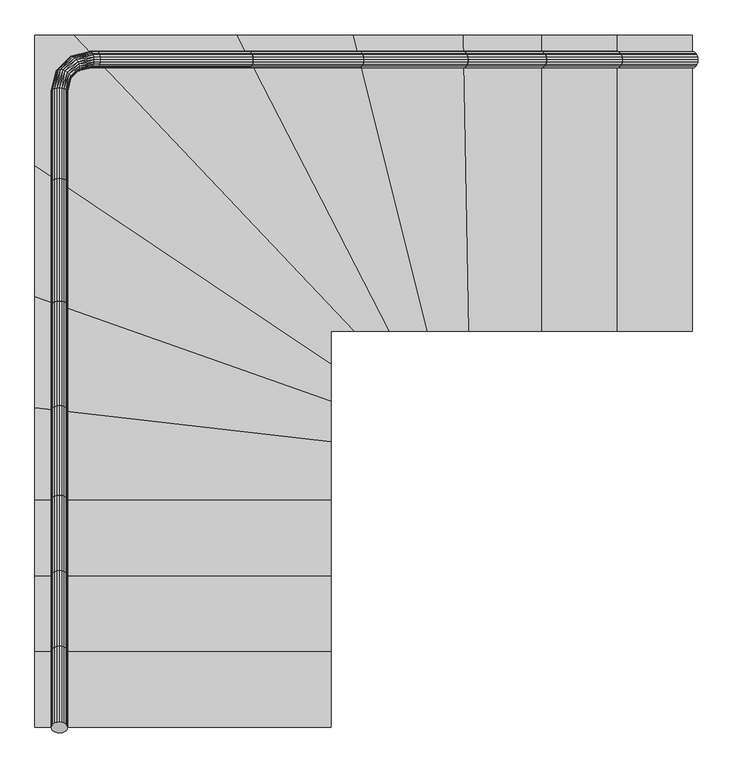
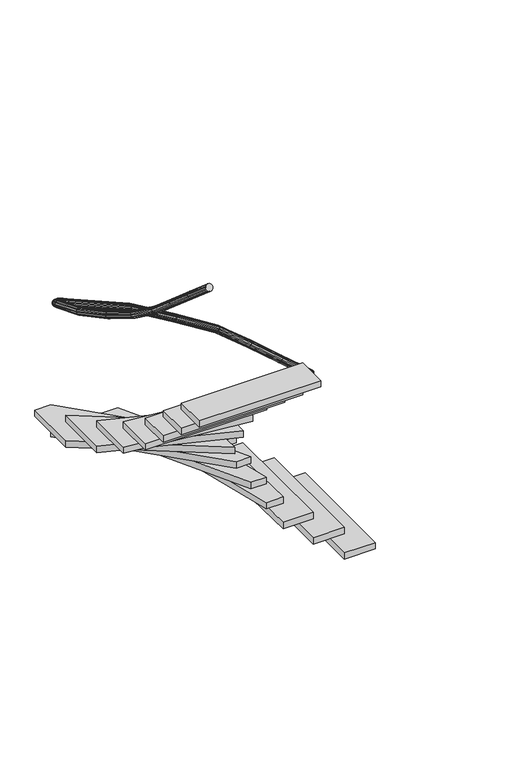
"""IFC4 building model written with IfcOpenShell, lengths in millimetres: stair geometry, 0_3d_modell."""

from ifc_helpers import new_model, si_unit, frame, origin, origin_with_axes, place, context, project, spatial, polyline, outline, extrude, faceted_brep, source, transform, mapped, element, save


def stair_5a7e43e8(model_context):
    return source(origin(), model_context, "Body", "SolidModel", [
        extrude(outline(polyline([(0.0, 988.8933271), (900.0, 884.9103911), (900.0, 706.9018591), (0.0, 706.9018591), (0.0, 988.8933271)])), frame((0.0, 0.0, 1787.1428571), z_axis=(0.0, 0.0, 1.0), x_axis=(1.0, 0.0, 0.0)), (0.0, 0.0, 1.0), 50.0),
        extrude(outline(polyline([(1.2235871, -7.9923214), (0.0, 0.0), (1.2235871, 7.9923214), (4.7745751, 15.2022986), (10.3053687, 20.924169), (17.2745751, 24.597836), (25.0, 25.8636953), (32.7254249, 24.597836), (39.6946313, 20.924169), (45.2254249, 15.2022986), (48.7764129, 7.9923214), (50.0, 0.0), (48.7764129, -7.9923214), (45.2254249, -15.2022986), (39.6946313, -20.924169), (32.7254249, -24.5978359), (25.0, -25.8636953), (17.2745751, -24.5978359), (10.3053687, -20.924169), (4.7745751, -15.2022986), (1.2235871, -7.9923214)])), frame((100.0, 246.9018591, 3252.4163795), z_axis=(0.0, -0.7569287102856999, 0.653497457948558), x_axis=(-1.0, 0.0, 0.0)), (0.0, 0.0, 1.0), 303.8595272),
        faceted_brep([(1775.2229617, 2022.7272828, 1074.1802827), (1770.0, 2021.5036957, 1068.1306652), (1764.7770383, 2022.7272828, 1062.0810477), (1760.0653365, 2026.2782709, 1056.6236089), (1756.3261087, 2031.8090644, 1052.2925609), (1753.9253768, 2038.7782709, 1049.511857), (1753.0981409, 2046.5036957, 1048.5536917), (1753.9253768, 2054.2291206, 1049.511857), (1756.3261087, 2061.198327, 1052.2925609), (1760.0653365, 2066.7291206, 1056.6236089), (1764.7770383, 2070.2801086, 1062.0810477), (1770.0, 2071.5036957, 1068.1306652), (1775.2229617, 2070.2801086, 1074.1802827), (1779.9346635, 2066.7291206, 1079.6377215), (1783.6738913, 2061.198327, 1083.9687694), (1786.0746232, 2054.2291206, 1086.7494734), (1786.9018591, 2046.5036957, 1087.7076387), (1786.0746232, 2038.7782709, 1086.7494734), (1783.6738913, 2031.8090644, 1083.9687694), (1779.9346635, 2026.2782709, 1079.6377215), (1534.8199564, 2022.7272828, 1260.6154227), (1540.0, 2021.5036957, 1266.7020937), (1545.1800436, 2022.7272828, 1272.7887648), (1549.8530284, 2026.2782709, 1278.2796301), (1553.5615302, 2031.8090644, 1282.6372054), (1555.9425348, 2038.7782709, 1285.434941), (1556.7629732, 2046.5036957, 1286.398975), (1555.9425348, 2054.2291206, 1285.434941), (1553.5615302, 2061.198327, 1282.6372054), (1549.8530284, 2066.7291206, 1278.2796301), (1545.1800436, 2070.2801086, 1272.7887648), (1540.0, 2071.5036957, 1266.7020937), (1534.8199564, 2070.2801086, 1260.6154227), (1530.1469716, 2066.7291206, 1255.1245574), (1526.4384698, 2061.198327, 1250.7669821), (1524.0574652, 2054.2291206, 1247.9692465), (1523.2370268, 2046.5036957, 1247.0052125), (1524.0574652, 2038.7782709, 1247.9692465), (1526.4384698, 2031.8090644, 1250.7669821), (1530.1469716, 2026.2782709, 1255.1245574)], [[[0, 1, 2, 3, 4, 5, 6, 7, 8, 9, 10, 11, 12, 13, 14, 15, 16, 17, 18, 19]], [[20, 21, 22, 23, 24, 25, 26, 27, 28, 29, 30, 31, 32, 33, 34, 35, 36, 37, 38, 39]], [[21, 1, 0, 22]], [[22, 0, 19, 23]], [[23, 19, 18, 24]], [[24, 18, 17, 25]], [[25, 17, 16, 26]], [[26, 16, 15, 27]], [[27, 15, 14, 28]], [[28, 14, 13, 29]], [[29, 13, 12, 30]], [[30, 12, 11, 31]], [[31, 11, 10, 32]], [[32, 10, 9, 33]], [[33, 9, 8, 34]], [[34, 8, 7, 35]], [[35, 7, 6, 36]], [[36, 6, 5, 37]], [[37, 5, 4, 38]], [[38, 4, 3, 39]], [[39, 3, 2, 20]], [[20, 2, 1, 21]]]),
        extrude(outline(polyline([(0.0, 246.9018591), (900.0, 246.9018591), (900.0, 16.9018591), (0.0, 16.9018591), (0.0, 246.9018591)])), frame((0.0, 0.0, 2382.8571429), z_axis=(0.0, 0.0, 1.0), x_axis=(1.0, 0.0, 0.0)), (0.0, 0.0, 1.0), 50.0),
        extrude(outline(polyline([(1770.0, 2121.5036957), (1770.0, 1221.5036957), (1540.0, 1221.5036957), (1540.0, 2121.5036957), (1770.0, 2121.5036957)])), frame((0.0, 0.0, 198.5714286), z_axis=(0.0, 0.0, 1.0), x_axis=(1.0, 0.0, 0.0)), (0.0, 0.0, 1.0), 50.0),
        extrude(outline(polyline([(0.0, 1326.2140709), (900.0, 1007.5896473), (900.0, 884.9103911), (0.0, 988.8933271), (0.0, 1326.2140709)])), frame((0.0, 0.0, 1588.5714286), z_axis=(0.0, 0.0, 1.0), x_axis=(1.0, 0.0, 0.0)), (0.0, 0.0, 1.0), 50.0),
        extrude(outline(polyline([(967.6813255, 2121.5036957), (1192.3186745, 1221.5036957), (1077.419675, 1221.5036957), (613.6390668, 2121.5036957), (967.6813255, 2121.5036957)])), frame((0.0, 0.0, 794.2857143), z_axis=(0.0, 0.0, 1.0), x_axis=(1.0, 0.0, 0.0)), (0.0, 0.0, 1.0), 50.0),
        extrude(outline(polyline([(0.0, 476.9018591), (900.0, 476.9018591), (900.0, 246.9018591), (0.0, 246.9018591), (0.0, 476.9018591)])), frame((0.0, 0.0, 2184.2857143), z_axis=(0.0, 0.0, 1.0), x_axis=(1.0, 0.0, 0.0)), (0.0, 0.0, 1.0), 50.0),
        extrude(outline(polyline([(1.2235871, -7.9923214), (0.0, 0.0), (1.2235871, 7.9923214), (4.7745751, 15.2022986), (10.3053687, 20.924169), (17.2745751, 24.5978359), (25.0, 25.8636953), (32.7254249, 24.5978359), (39.6946313, 20.924169), (45.2254249, 15.2022986), (48.7764129, 7.9923214), (50.0, 0.0), (48.7764129, -7.9923214), (45.2254249, -15.2022986), (39.6946313, -20.9241691), (32.7254249, -24.5978359), (25.0, -25.8636953), (17.2745751, -24.5978359), (10.3053687, -20.9241691), (4.7745751, -15.2022986), (1.2235871, -7.9923214)])), frame((100.0, 476.9018591, 3053.8449509), z_axis=(0.0, -0.7569287102856925, 0.6534974579485664), x_axis=(-1.0, 0.0, 0.0)), (0.0, 0.0, 1.0), 303.8595272),
        extrude(outline(polyline([(1540.0, 2121.5036957), (1540.0, 1221.5036957), (1318.0495551, 1221.5036957), (1301.9504449, 2121.5036957), (1540.0, 2121.5036957)])), frame((0.0, 0.0, 397.1428571), z_axis=(0.0, 0.0, 1.0), x_axis=(1.0, 0.0, 0.0)), (0.0, 0.0, 1.0), 50.0),
        faceted_brep([(1545.1800436, 2022.7272828, 1272.7887648), (1540.0, 2021.5036957, 1266.7020937), (1534.8199564, 2022.7272828, 1260.6154227), (1530.1469716, 2026.2782709, 1255.1245574), (1526.4384698, 2031.8090644, 1250.7669821), (1524.0574652, 2038.7782709, 1247.9692465), (1523.2370268, 2046.5036957, 1247.0052125), (1524.0574652, 2054.2291206, 1247.9692465), (1526.4384698, 2061.198327, 1250.7669821), (1530.1469716, 2066.7291206, 1255.1245574), (1534.8199564, 2070.2801086, 1260.6154227), (1540.0, 2071.5036957, 1266.7020937), (1545.1800436, 2070.2801086, 1272.7887648), (1549.8530284, 2066.7291206, 1278.2796301), (1553.5615302, 2061.198327, 1282.6372054), (1555.9425348, 2054.2291206, 1285.434941), (1556.7629732, 2046.5036957, 1286.398975), (1555.9425348, 2038.7782709, 1285.434941), (1553.5615302, 2031.8090644, 1282.6372054), (1549.8530284, 2026.2782709, 1278.2796301), (1298.5793418, 2022.7272828, 1458.7947987), (1303.2920374, 2021.5036957, 1465.2735223), (1308.004733, 2022.7272828, 1471.7522459), (1312.2561171, 2026.2782709, 1477.5967869), (1315.6300346, 2031.8090644, 1482.2350408), (1317.796223, 2038.7782709, 1485.2129832), (1318.5426407, 2046.5036957, 1486.2391122), (1317.796223, 2054.2291206, 1485.2129832), (1315.6300346, 2061.198327, 1482.2350408), (1312.2561171, 2066.7291206, 1477.5967869), (1308.004733, 2070.2801086, 1471.7522459), (1303.2920374, 2071.5036957, 1465.2735223), (1298.5793418, 2070.2801086, 1458.7947987), (1294.3279577, 2066.7291206, 1452.9502578), (1290.9540401, 2061.198327, 1448.3120038), (1288.7878517, 2054.2291206, 1445.3340614), (1288.0414341, 2046.5036957, 1444.3079324), (1288.7878517, 2038.7782709, 1445.3340614), (1290.9540401, 2031.8090644, 1448.3120038), (1294.3279577, 2026.2782709, 1452.9502578)], [[[0, 1, 2, 3, 4, 5, 6, 7, 8, 9, 10, 11, 12, 13, 14, 15, 16, 17, 18, 19]], [[20, 21, 22, 23, 24, 25, 26, 27, 28, 29, 30, 31, 32, 33, 34, 35, 36, 37, 38, 39]], [[21, 1, 0, 22]], [[22, 0, 19, 23]], [[23, 19, 18, 24]], [[24, 18, 17, 25]], [[25, 17, 16, 26]], [[26, 16, 15, 27]], [[27, 15, 14, 28]], [[28, 14, 13, 29]], [[29, 13, 12, 30]], [[30, 12, 11, 31]], [[31, 11, 10, 32]], [[32, 10, 9, 33]], [[33, 9, 8, 34]], [[34, 8, 7, 35]], [[35, 7, 6, 36]], [[36, 6, 5, 37]], [[37, 5, 4, 38]], [[38, 4, 3, 39]], [[39, 3, 2, 20]], [[20, 2, 1, 21]]]),
        extrude(outline(polyline([(118.0988626, 2121.5036957), (970.0, 1221.5036957), (900.0, 1221.5036957), (900.0, 1121.5036957), (0.0, 1724.0707938), (0.0, 2121.5036957), (118.0988626, 2121.5036957)])), frame((0.0, 0.0, 1191.4285714), z_axis=(0.0, 0.0, 1.0), x_axis=(1.0, 0.0, 0.0)), (0.0, 0.0, 1.0), 50.0),
        extrude(outline(polyline([(1301.9504449, 2121.5036957), (1318.0495551, 1221.5036957), (1192.3186745, 1221.5036957), (967.6813255, 2121.5036957), (1301.9504449, 2121.5036957)])), frame((0.0, 0.0, 595.7142857), z_axis=(0.0, 0.0, 1.0), x_axis=(1.0, 0.0, 0.0)), (0.0, 0.0, 1.0), 50.0),
        extrude(outline(polyline([(613.6390668, 2121.5036957), (1077.419675, 1221.5036957), (970.0, 1221.5036957), (118.0988626, 2121.5036957), (613.6390668, 2121.5036957)])), frame((0.0, 0.0, 992.8571429), z_axis=(0.0, 0.0, 1.0), x_axis=(1.0, 0.0, 0.0)), (0.0, 0.0, 1.0), 50.0),
        faceted_brep([(98.7764129, 984.692421, 2663.3376045), (100.0, 980.2280824, 2656.7020937), (98.7764129, 975.7637439, 2650.066583), (95.2254249, 971.7364059, 2644.0806023), (89.6946313, 968.5402924, 2639.3301012), (82.7254249, 966.4882612, 2636.2800917), (75.0, 965.7811794, 2635.22913), (67.2745751, 966.4882612, 2636.2800917), (60.3053687, 968.5402924, 2639.3301012), (54.7745751, 971.7364059, 2644.0806023), (51.2235871, 975.7637439, 2650.066583), (50.0, 980.2280824, 2656.7020937), (51.2235871, 984.692421, 2663.3376045), (54.7745751, 988.719759, 2669.3235852), (60.3053687, 991.9158725, 2674.0740863), (67.2745751, 993.9679037, 2677.1240958), (75.0, 994.6749855, 2678.1750575), (82.7254249, 993.9679037, 2677.1240958), (89.6946313, 991.9158725, 2674.0740863), (95.2254249, 988.719759, 2669.3235852), (98.7764129, 701.932844, 2849.004659), (100.0, 706.9018591, 2855.2735223), (98.7764129, 711.8708742, 2861.5423857), (95.2254249, 716.3534875, 2867.197609), (89.6946313, 719.9109095, 2871.6856196), (82.7254249, 722.194915, 2874.5670998), (75.0, 722.9819297, 2875.5599903), (67.2745751, 722.194915, 2874.5670998), (60.3053687, 719.9109095, 2871.6856196), (54.7745751, 716.3534875, 2867.197609), (51.2235871, 711.8708742, 2861.5423857), (50.0, 706.9018591, 2855.2735223), (51.2235871, 701.932844, 2849.004659), (54.7745751, 697.4502308, 2843.3494356), (60.3053687, 693.8928087, 2838.861425), (67.2745751, 691.6088032, 2835.9799448), (75.0, 690.8217885, 2834.9870544), (82.7254249, 691.6088032, 2835.9799448), (89.6946313, 693.8928087, 2838.861425), (95.2254249, 697.4502308, 2843.3494356)], [[[0, 1, 2, 3, 4, 5, 6, 7, 8, 9, 10, 11, 12, 13, 14, 15, 16, 17, 18, 19]], [[20, 21, 22, 23, 24, 25, 26, 27, 28, 29, 30, 31, 32, 33, 34, 35, 36, 37, 38, 39]], [[21, 1, 0, 22]], [[22, 0, 19, 23]], [[23, 19, 18, 24]], [[24, 18, 17, 25]], [[25, 17, 16, 26]], [[26, 16, 15, 27]], [[27, 15, 14, 28]], [[28, 14, 13, 29]], [[29, 13, 12, 30]], [[30, 12, 11, 31]], [[31, 11, 10, 32]], [[32, 10, 9, 33]], [[33, 9, 8, 34]], [[34, 8, 7, 35]], [[35, 7, 6, 36]], [[36, 6, 5, 37]], [[37, 5, 4, 38]], [[38, 4, 3, 39]], [[39, 3, 2, 20]], [[20, 2, 1, 21]]]),
        faceted_brep([(98.7764129, 1677.2481385, 2266.8075559), (100.0, 1673.856869, 2259.5592366), (98.7764129, 1670.4655995, 2252.3109173), (95.2254249, 1667.4062911, 2245.772114), (89.6946313, 1664.9784102, 2240.5828904), (82.7254249, 1663.4196147, 2237.2512037), (75.0, 1662.8824904, 2236.1031827), (67.2745751, 1663.4196147, 2237.2512037), (60.3053687, 1664.9784102, 2240.5828904), (54.7745751, 1667.4062911, 2245.772114), (51.2235871, 1670.4655995, 2252.3109173), (50.0, 1673.856869, 2259.5592366), (51.2235871, 1677.2481385, 2266.8075559), (54.7745751, 1680.3074469, 2273.3463592), (60.3053687, 1682.7353278, 2278.5355829), (67.2745751, 1684.2941233, 2281.8672695), (75.0, 1684.8312476, 2283.0152905), (82.7254249, 1684.2941233, 2281.8672695), (89.6946313, 1682.7353278, 2278.5355829), (95.2254249, 1680.3074469, 2273.3463592), (98.7764129, 1295.6744399, 2451.1987943), (100.0, 1299.6620356, 2458.1306652), (98.7764129, 1303.6496314, 2465.062536), (95.2254249, 1307.2468935, 2471.3158671), (89.6946313, 1310.1016969, 2476.2785387), (82.7254249, 1311.9345935, 2479.46477), (75.0, 1312.5661666, 2480.5626705), (67.2745751, 1311.9345935, 2479.46477), (60.3053687, 1310.1016969, 2476.2785387), (54.7745751, 1307.2468935, 2471.3158671), (51.2235871, 1303.6496314, 2465.062536), (50.0, 1299.6620356, 2458.1306652), (51.2235871, 1295.6744399, 2451.1987943), (54.7745751, 1292.0771778, 2444.9454632), (60.3053687, 1289.2223744, 2439.9827916), (67.2745751, 1287.3894778, 2436.7965603), (75.0, 1286.7579047, 2435.6986598), (82.7254249, 1287.3894778, 2436.7965603), (89.6946313, 1289.2223744, 2439.9827916), (95.2254249, 1292.0771778, 2444.9454632)], [[[0, 1, 2, 3, 4, 5, 6, 7, 8, 9, 10, 11, 12, 13, 14, 15, 16, 17, 18, 19]], [[20, 21, 22, 23, 24, 25, 26, 27, 28, 29, 30, 31, 32, 33, 34, 35, 36, 37, 38, 39]], [[21, 1, 0, 22]], [[22, 0, 19, 23]], [[23, 19, 18, 24]], [[24, 18, 17, 25]], [[25, 17, 16, 26]], [[26, 16, 15, 27]], [[27, 15, 14, 28]], [[28, 14, 13, 29]], [[29, 13, 12, 30]], [[30, 12, 11, 31]], [[31, 11, 10, 32]], [[32, 10, 9, 33]], [[33, 9, 8, 34]], [[34, 8, 7, 35]], [[35, 7, 6, 36]], [[36, 6, 5, 37]], [[37, 5, 4, 38]], [[38, 4, 3, 39]], [[39, 3, 2, 20]], [[20, 2, 1, 21]]]),
        faceted_brep([(98.7764129, 1303.6496314, 2465.062536), (100.0, 1299.6620356, 2458.1306652), (98.7764129, 1295.6744399, 2451.1987943), (95.2254249, 1292.0771778, 2444.9454632), (89.6946313, 1289.2223744, 2439.9827916), (82.7254249, 1287.3894778, 2436.7965603), (75.0, 1286.7579047, 2435.6986598), (67.2745751, 1287.3894778, 2436.7965603), (60.3053687, 1289.2223744, 2439.9827916), (54.7745751, 1292.0771778, 2444.9454632), (51.2235871, 1295.6744399, 2451.1987943), (50.0, 1299.6620356, 2458.1306652), (51.2235871, 1303.6496314, 2465.062536), (54.7745751, 1307.2468935, 2471.3158671), (60.3053687, 1310.1016969, 2476.2785387), (67.2745751, 1311.9345935, 2479.46477), (75.0, 1312.5661666, 2480.5626705), (82.7254249, 1311.9345935, 2479.46477), (89.6946313, 1310.1016969, 2476.2785387), (95.2254249, 1307.2468935, 2471.3158671), (98.7764129, 975.7637439, 2650.066583), (100.0, 980.2280824, 2656.7020937), (98.7764129, 984.692421, 2663.3376045), (95.2254249, 988.719759, 2669.3235852), (89.6946313, 991.9158725, 2674.0740863), (82.7254249, 993.9679037, 2677.1240958), (75.0, 994.6749855, 2678.1750575), (67.2745751, 993.9679037, 2677.1240958), (60.3053687, 991.9158725, 2674.0740863), (54.7745751, 988.719759, 2669.3235852), (51.2235871, 984.692421, 2663.3376045), (50.0, 980.2280824, 2656.7020937), (51.2235871, 975.7637439, 2650.066583), (54.7745751, 971.7364059, 2644.0806023), (60.3053687, 968.5402924, 2639.3301012), (67.2745751, 966.4882612, 2636.2800917), (75.0, 965.7811794, 2635.22913), (82.7254249, 966.4882612, 2636.2800917), (89.6946313, 968.5402924, 2639.3301012), (95.2254249, 971.7364059, 2644.0806023)], [[[0, 1, 2, 3, 4, 5, 6, 7, 8, 9, 10, 11, 12, 13, 14, 15, 16, 17, 18, 19]], [[20, 21, 22, 23, 24, 25, 26, 27, 28, 29, 30, 31, 32, 33, 34, 35, 36, 37, 38, 39]], [[21, 1, 0, 22]], [[22, 0, 19, 23]], [[23, 19, 18, 24]], [[24, 18, 17, 25]], [[25, 17, 16, 26]], [[26, 16, 15, 27]], [[27, 15, 14, 28]], [[28, 14, 13, 29]], [[29, 13, 12, 30]], [[30, 12, 11, 31]], [[31, 11, 10, 32]], [[32, 10, 9, 33]], [[33, 9, 8, 34]], [[34, 8, 7, 35]], [[35, 7, 6, 36]], [[36, 6, 5, 37]], [[37, 5, 4, 38]], [[38, 4, 3, 39]], [[39, 3, 2, 20]], [[20, 2, 1, 21]]]),
        extrude(outline(polyline([(1.2235871, -7.9923214), (0.0, 0.0), (1.2235871, 7.9923214), (4.7745752, 15.2022986), (10.3053687, 20.9241691), (17.2745752, 24.5978359), (25.0, 25.8636953), (32.7254249, 24.5978359), (39.6946313, 20.9241691), (45.2254249, 15.2022986), (48.7764129, 7.9923214), (50.0, 0.0), (48.7764129, -7.9923214), (45.2254249, -15.2022986), (39.6946313, -20.9241691), (32.7254249, -24.5978359), (25.0, -25.8636953), (17.2745752, -24.5978359), (10.3053687, -20.9241691), (4.7745752, -15.2022986), (1.2235871, -7.9923214)])), frame((2000.0, 2021.5036957, 869.5592366), z_axis=(-0.7569287102857621, 0.0, 0.6534974579484858), x_axis=(0.0, 1.0, 0.0)), (0.0, 0.0, 1.0), 303.8595272),
        faceted_brep([(98.7764129, 711.8708742, 2861.5423857), (100.0, 706.9018591, 2855.2735223), (98.7764129, 701.932844, 2849.004659), (95.2254249, 697.4502308, 2843.3494356), (89.6946313, 693.8928087, 2838.861425), (82.7254249, 691.6088032, 2835.9799448), (75.0, 690.8217885, 2834.9870544), (67.2745751, 691.6088032, 2835.9799448), (60.3053687, 693.8928087, 2838.861425), (54.7745751, 697.4502308, 2843.3494356), (51.2235871, 701.932844, 2849.004659), (50.0, 706.9018591, 2855.2735223), (51.2235871, 711.8708742, 2861.5423857), (54.7745751, 716.3534875, 2867.197609), (60.3053687, 719.9109095, 2871.6856196), (67.2745751, 722.194915, 2874.5670998), (75.0, 722.9819297, 2875.5599903), (82.7254249, 722.194915, 2874.5670998), (89.6946313, 719.9109095, 2871.6856196), (95.2254249, 716.3534875, 2867.197609), (98.7764129, 471.6788974, 3047.7953334), (100.0, 476.9018591, 3053.8449509), (98.7764129, 482.1248208, 3059.8945684), (95.2254249, 486.8365226, 3065.3520072), (89.6946313, 490.5757504, 3069.6830552), (82.7254249, 492.9764824, 3072.4637591), (75.0, 493.8037182, 3073.4219244), (67.2745751, 492.9764824, 3072.4637591), (60.3053687, 490.5757504, 3069.6830552), (54.7745751, 486.8365226, 3065.3520072), (51.2235871, 482.1248208, 3059.8945684), (50.0, 476.9018591, 3053.8449509), (51.2235871, 471.6788974, 3047.7953334), (54.7745751, 466.9671956, 3042.3378946), (60.3053687, 463.2279679, 3038.0068466), (67.2745751, 460.8272359, 3035.2261427), (75.0, 460.0, 3034.2679774), (82.7254249, 460.8272359, 3035.2261427), (89.6946313, 463.2279679, 3038.0068466), (95.2254249, 466.9671956, 3042.3378946)], [[[0, 1, 2, 3, 4, 5, 6, 7, 8, 9, 10, 11, 12, 13, 14, 15, 16, 17, 18, 19]], [[20, 21, 22, 23, 24, 25, 26, 27, 28, 29, 30, 31, 32, 33, 34, 35, 36, 37, 38, 39]], [[21, 1, 0, 22]], [[22, 0, 19, 23]], [[23, 19, 18, 24]], [[24, 18, 17, 25]], [[25, 17, 16, 26]], [[26, 16, 15, 27]], [[27, 15, 14, 28]], [[28, 14, 13, 29]], [[29, 13, 12, 30]], [[30, 12, 11, 31]], [[31, 11, 10, 32]], [[32, 10, 9, 33]], [[33, 9, 8, 34]], [[34, 8, 7, 35]], [[35, 7, 6, 36]], [[36, 6, 5, 37]], [[37, 5, 4, 38]], [[38, 4, 3, 39]], [[39, 3, 2, 20]], [[20, 2, 1, 21]]]),
        extrude(outline(polyline([(0.0, 706.9018591), (900.0, 706.9018591), (900.0, 476.9018591), (0.0, 476.9018591), (0.0, 706.9018591)])), frame((0.0, 0.0, 1985.7142857), z_axis=(0.0, 0.0, 1.0), x_axis=(1.0, 0.0, 0.0)), (0.0, 0.0, 1.0), 50.0),
        faceted_brep([(990.5652448, 2022.7272828, 1670.6674124), (986.4011046, 2021.5036957, 1663.8449509), (982.2369643, 2022.7272828, 1657.0224894), (978.4804392, 2026.2782709, 1650.867858), (975.4992439, 2031.8090644, 1645.9835149), (973.5851987, 2038.7782709, 1642.8475735), (972.9256637, 2046.5036957, 1641.7670018), (973.5851987, 2054.2291206, 1642.8475735), (975.4992439, 2061.198327, 1645.9835149), (978.4804392, 2066.7291206, 1650.867858), (982.2369643, 2070.2801086, 1657.0224894), (986.4011046, 2071.5036957, 1663.8449509), (990.5652448, 2070.2801086, 1670.6674124), (994.32177, 2066.7291206, 1676.8220438), (997.3029652, 2061.198327, 1681.7063869), (999.2170104, 2054.2291206, 1684.8423282), (999.8765454, 2046.5036957, 1685.9229), (999.2170104, 2038.7782709, 1684.8423282), (997.3029652, 2031.8090644, 1681.7063869), (994.32177, 2026.2782709, 1676.8220438), (648.6556288, 2022.7272828, 1855.277549), (652.2874508, 2021.5036957, 1862.4163795), (655.9192729, 2022.7272828, 1869.5552099), (659.1955868, 2026.2782709, 1875.9952419), (661.7956843, 2031.8090644, 1881.1060802), (663.4650497, 2038.7782709, 1884.3874404), (664.0402738, 2046.5036957, 1885.51812), (663.4650497, 2054.2291206, 1884.3874404), (661.7956843, 2061.198327, 1881.1060802), (659.1955868, 2066.7291206, 1875.9952419), (655.9192729, 2070.2801086, 1869.5552099), (652.2874508, 2071.5036957, 1862.4163795), (648.6556288, 2070.2801086, 1855.277549), (645.3793148, 2066.7291206, 1848.8375171), (642.7792174, 2061.198327, 1843.7266788), (641.109852, 2054.2291206, 1840.4453186), (640.5346279, 2046.5036957, 1839.3146389), (641.109852, 2038.7782709, 1840.4453186), (642.7792174, 2031.8090644, 1843.7266788), (645.3793148, 2026.2782709, 1848.8375171)], [[[0, 1, 2, 3, 4, 5, 6, 7, 8, 9, 10, 11, 12, 13, 14, 15, 16, 17, 18, 19]], [[20, 21, 22, 23, 24, 25, 26, 27, 28, 29, 30, 31, 32, 33, 34, 35, 36, 37, 38, 39]], [[21, 1, 0, 22]], [[22, 0, 19, 23]], [[23, 19, 18, 24]], [[24, 18, 17, 25]], [[25, 17, 16, 26]], [[26, 16, 15, 27]], [[27, 15, 14, 28]], [[28, 14, 13, 29]], [[29, 13, 12, 30]], [[30, 12, 11, 31]], [[31, 11, 10, 32]], [[32, 10, 9, 33]], [[33, 9, 8, 34]], [[34, 8, 7, 35]], [[35, 7, 6, 36]], [[36, 6, 5, 37]], [[37, 5, 4, 38]], [[38, 4, 3, 39]], [[39, 3, 2, 20]], [[20, 2, 1, 21]]]),
        faceted_brep([(192.1749264, 2022.7272828, 2068.3613589), (189.0906241, 2021.5036957, 2060.987808), (186.0063217, 2022.7272828, 2053.6142572), (183.2239324, 2026.2782709, 2046.9624808), (181.0158157, 2031.8090644, 2041.6836012), (179.5981175, 2038.7782709, 2038.2943519), (179.109612, 2046.5036957, 2037.1264962), (179.5981175, 2054.2291206, 2038.2943519), (181.0158157, 2061.198327, 2041.6836012), (183.2239324, 2066.7291206, 2046.9624808), (186.0063217, 2070.2801086, 2053.6142572), (189.0906241, 2071.5036957, 2060.987808), (192.1749264, 2070.2801086, 2068.3613589), (194.9573158, 2066.7291206, 2075.0131352), (197.1654325, 2061.198327, 2080.2920148), (198.5831307, 2054.2291206, 2083.6812642), (199.0716362, 2046.5036957, 2084.8491199), (198.5831307, 2038.7782709, 2083.6812642), (197.1654325, 2031.8090644, 2080.2920148), (194.9573158, 2026.2782709, 2075.0131352), (98.7764129, 1670.4655995, 2252.3109173), (100.0, 1673.856869, 2259.5592366), (98.7764129, 1677.2481385, 2266.8075559), (95.2254249, 1680.3074469, 2273.3463592), (89.6946313, 1682.7353278, 2278.5355829), (82.7254249, 1684.2941233, 2281.8672695), (75.0, 1684.8312476, 2283.0152905), (67.2745751, 1684.2941233, 2281.8672695), (60.3053687, 1682.7353278, 2278.5355829), (54.7745751, 1680.3074469, 2273.3463592), (51.2235871, 1677.2481385, 2266.8075559), (50.0, 1673.856869, 2259.5592366), (51.2235871, 1670.4655995, 2252.3109173), (54.7745751, 1667.4062911, 2245.772114), (60.3053687, 1664.9784102, 2240.5828904), (67.2745751, 1663.4196147, 2237.2512037), (75.0, 1662.8824904, 2236.1031827), (82.7254249, 1663.4196147, 2237.2512037), (89.6946313, 1664.9784102, 2240.5828904), (95.2254249, 1667.4062911, 2245.772114), (170.7900373, 2021.5036957, 2068.4537913), (173.8090484, 2022.7272828, 2075.8539787), (176.5325377, 2026.2782709, 2082.5297841), (178.693911, 2031.8090644, 2087.8277333), (180.0815981, 2038.7782709, 2091.2292261), (180.5597625, 2046.5036957, 2092.4013006), (180.0815981, 2054.2291206, 2091.2292261), (178.693911, 2061.198327, 2087.8277333), (176.5325377, 2066.7291206, 2082.5297841), (173.8090484, 2070.2801086, 2075.8539787), (170.7900373, 2071.5036957, 2068.4537913), (167.7710262, 2070.2801086, 2061.053604), (165.0475369, 2066.7291206, 2054.3777985), (162.8861636, 2061.198327, 2049.0798493), (161.4984765, 2054.2291206, 2045.6783565), (161.0203121, 2046.5036957, 2044.506282), (161.4984765, 2038.7782709, 2045.6783565), (162.8861636, 2031.8090644, 2049.0798493), (165.0475369, 2026.2782709, 2054.3777985), (167.7710262, 2022.7272828, 2061.053604), (132.2001384, 2012.6032946, 2093.9682441), (135.0103672, 2015.5333905, 2100.9604911), (136.3719857, 2020.3241085, 2107.2682883), (136.1517092, 2026.5064996, 2112.2741844), (134.3710999, 2033.4753883, 2115.4881676), (131.2044563, 2040.5486112, 2116.5956307), (126.9617515, 2047.0337921, 2115.4881676), (122.058291, 2052.2961161, 2112.2741844), (116.9740597, 2055.8204705, 2107.2682883), (112.2067376, 2057.2618667, 2100.9604911), (108.2229833, 2056.4792109, 2093.9682441), (105.4127546, 2053.549115, 2086.9759971), (104.0511361, 2048.758397, 2080.6681999), (104.2714126, 2042.5760059, 2075.6623037), (106.0520218, 2035.6071172, 2072.4483206), (109.2186654, 2028.5338943, 2071.3408574), (113.4613702, 2022.0487134, 2072.4483206), (118.3648307, 2016.7863894, 2075.6623037), (123.449062, 2013.262035, 2080.6681999), (128.2163841, 2011.8206388, 2086.9759971), (108.9004011, 1989.3035573, 2121.0971401), (109.6830569, 1993.2873116, 2128.0893871), (108.2416607, 1998.0546337, 2134.3971843), (104.7173064, 2003.138865, 2139.4030804), (99.4549823, 2008.0423255, 2142.6170636), (92.9698015, 2012.2850303, 2143.7245267), (85.8965785, 2015.4516739, 2142.6170636), (78.9276898, 2017.2322831, 2139.4030804), (72.7452987, 2017.4525596, 2134.3971843), (67.9545808, 2016.0909411, 2128.0893871), (65.0244848, 2013.2807124, 2121.0971401), (64.241829, 2009.2969581, 2114.1048931), (65.6832253, 2004.529636, 2107.7970959), (69.2075796, 1999.4454047, 2102.7911997), (74.4699036, 1994.5419442, 2099.5772166), (80.9550845, 1990.2992394, 2098.4697534), (88.0283074, 1987.1325958, 2099.5772166), (94.9971961, 1985.3519865, 2102.7911997), (101.1795872, 1985.1317101, 2107.7970959), (105.9703052, 1986.4933285, 2114.1048931), (100.0, 1950.7136584, 2146.6115929), (98.7764129, 1953.7326696, 2154.0117802), (95.2254249, 1956.4561588, 2160.6875857), (89.6946313, 1958.6175321, 2165.9855349), (82.7254249, 1960.0052192, 2169.3870277), (75.0, 1960.4833836, 2170.5591022), (67.2745751, 1960.0052192, 2169.3870277), (60.3053687, 1958.6175321, 2165.9855349), (54.7745751, 1956.4561588, 2160.6875857), (51.2235871, 1953.7326696, 2154.0117802), (50.0, 1950.7136584, 2146.6115929), (51.2235871, 1947.6946473, 2139.2114055), (54.7745751, 1944.971158, 2132.5356001), (60.3053687, 1942.8097847, 2127.2376509), (67.2745751, 1941.4220976, 2123.8361581), (75.0, 1940.9439332, 2122.6640835), (82.7254249, 1941.4220976, 2123.8361581), (89.6946313, 1942.8097847, 2127.2376509), (95.2254249, 1944.971158, 2132.5356001), (98.7764129, 1947.6946473, 2139.2114055)], [[[0, 1, 2, 3, 4, 5, 6, 7, 8, 9, 10, 11, 12, 13, 14, 15, 16, 17, 18, 19]], [[20, 21, 22, 23, 24, 25, 26, 27, 28, 29, 30, 31, 32, 33, 34, 35, 36, 37, 38, 39]], [[40, 1, 0, 41]], [[41, 0, 19, 42]], [[42, 19, 18, 43]], [[43, 18, 17, 44]], [[44, 17, 16, 45]], [[45, 16, 15, 46]], [[46, 15, 14, 47]], [[47, 14, 13, 48]], [[48, 13, 12, 49]], [[49, 12, 11, 50]], [[50, 11, 10, 51]], [[51, 10, 9, 52]], [[52, 9, 8, 53]], [[53, 8, 7, 54]], [[54, 7, 6, 55]], [[55, 6, 5, 56]], [[56, 5, 4, 57]], [[57, 4, 3, 58]], [[58, 3, 2, 59]], [[59, 2, 1, 40]], [[60, 40, 41]], [[60, 41, 61]], [[61, 41, 42]], [[61, 42, 62]], [[62, 42, 43]], [[62, 43, 63]], [[63, 43, 44]], [[63, 44, 64]], [[64, 44, 45]], [[64, 45, 65]], [[65, 45, 46]], [[65, 46, 66]], [[66, 46, 47]], [[66, 47, 67]], [[67, 47, 48]], [[67, 48, 68]], [[68, 48, 49]], [[68, 49, 69]], [[69, 49, 50]], [[69, 50, 70]], [[70, 50, 51]], [[70, 51, 71]], [[71, 51, 52]], [[71, 52, 72]], [[72, 52, 53]], [[72, 53, 73]], [[73, 53, 54]], [[73, 54, 74]], [[74, 54, 55]], [[74, 55, 75]], [[75, 55, 56]], [[75, 56, 76]], [[76, 56, 57]], [[76, 57, 77]], [[77, 57, 58]], [[77, 58, 78]], [[78, 58, 59]], [[78, 59, 79]], [[79, 59, 40]], [[79, 40, 60]], [[80, 60, 61]], [[80, 61, 81]], [[81, 61, 62]], [[81, 62, 82]], [[82, 62, 63]], [[82, 63, 83]], [[83, 63, 64]], [[83, 64, 84]], [[84, 64, 65]], [[84, 65, 85]], [[85, 65, 66]], [[85, 66, 86]], [[86, 66, 67]], [[86, 67, 87]], [[87, 67, 68]], [[87, 68, 88]], [[88, 68, 69]], [[88, 69, 89]], [[89, 69, 70]], [[89, 70, 90]], [[90, 70, 71]], [[90, 71, 91]], [[91, 71, 72]], [[91, 72, 92]], [[92, 72, 73]], [[92, 73, 93]], [[93, 73, 74]], [[93, 74, 94]], [[94, 74, 75]], [[94, 75, 95]], [[95, 75, 76]], [[95, 76, 96]], [[96, 76, 77]], [[96, 77, 97]], [[97, 77, 78]], [[97, 78, 98]], [[98, 78, 79]], [[98, 79, 99]], [[99, 79, 60]], [[99, 60, 80]], [[100, 80, 81]], [[100, 81, 101]], [[101, 81, 82]], [[101, 82, 102]], [[102, 82, 83]], [[102, 83, 103]], [[103, 83, 84]], [[103, 84, 104]], [[104, 84, 85]], [[104, 85, 105]], [[105, 85, 86]], [[105, 86, 106]], [[106, 86, 87]], [[106, 87, 107]], [[107, 87, 88]], [[107, 88, 108]], [[108, 88, 89]], [[108, 89, 109]], [[109, 89, 90]], [[109, 90, 110]], [[110, 90, 91]], [[110, 91, 111]], [[111, 91, 92]], [[111, 92, 112]], [[112, 92, 93]], [[112, 93, 113]], [[113, 93, 94]], [[113, 94, 114]], [[114, 94, 95]], [[114, 95, 115]], [[115, 95, 96]], [[115, 96, 116]], [[116, 96, 97]], [[116, 97, 117]], [[117, 97, 98]], [[117, 98, 118]], [[118, 98, 99]], [[118, 99, 119]], [[119, 99, 80]], [[119, 80, 100]], [[21, 100, 101, 22]], [[22, 101, 102, 23]], [[23, 102, 103, 24]], [[24, 103, 104, 25]], [[25, 104, 105, 26]], [[26, 105, 106, 27]], [[27, 106, 107, 28]], [[28, 107, 108, 29]], [[29, 108, 109, 30]], [[30, 109, 110, 31]], [[31, 110, 111, 32]], [[32, 111, 112, 33]], [[33, 112, 113, 34]], [[34, 113, 114, 35]], [[35, 114, 115, 36]], [[36, 115, 116, 37]], [[37, 116, 117, 38]], [[38, 117, 118, 39]], [[39, 118, 119, 20]], [[20, 119, 100, 21]]]),
        faceted_brep([(1308.004733, 2022.7272828, 1471.7522459), (1303.2920374, 2021.5036957, 1465.2735223), (1298.5793418, 2022.7272828, 1458.7947987), (1294.3279577, 2026.2782709, 1452.9502578), (1290.9540401, 2031.8090644, 1448.3120038), (1288.7878517, 2038.7782709, 1445.3340614), (1288.0414341, 2046.5036957, 1444.3079324), (1288.7878517, 2054.2291206, 1445.3340614), (1290.9540401, 2061.198327, 1448.3120038), (1294.3279577, 2066.7291206, 1452.9502578), (1298.5793418, 2070.2801086, 1458.7947987), (1303.2920374, 2071.5036957, 1465.2735223), (1308.004733, 2070.2801086, 1471.7522459), (1312.2561171, 2066.7291206, 1477.5967869), (1315.6300346, 2061.198327, 1482.2350408), (1317.796223, 2054.2291206, 1485.2129832), (1318.5426407, 2046.5036957, 1486.2391122), (1317.796223, 2038.7782709, 1485.2129832), (1315.6300346, 2031.8090644, 1482.2350408), (1312.2561171, 2026.2782709, 1477.5967869), (982.2369643, 2022.7272828, 1657.0224894), (986.4011046, 2021.5036957, 1663.8449509), (990.5652448, 2022.7272828, 1670.6674124), (994.32177, 2026.2782709, 1676.8220438), (997.3029652, 2031.8090644, 1681.7063869), (999.2170104, 2038.7782709, 1684.8423282), (999.8765454, 2046.5036957, 1685.9229), (999.2170104, 2054.2291206, 1684.8423282), (997.3029652, 2061.198327, 1681.7063869), (994.32177, 2066.7291206, 1676.8220438), (990.5652448, 2070.2801086, 1670.6674124), (986.4011046, 2071.5036957, 1663.8449509), (982.2369643, 2070.2801086, 1657.0224894), (978.4804392, 2066.7291206, 1650.867858), (975.4992439, 2061.198327, 1645.9835149), (973.5851987, 2054.2291206, 1642.8475735), (972.9256637, 2046.5036957, 1641.7670018), (973.5851987, 2038.7782709, 1642.8475735), (975.4992439, 2031.8090644, 1645.9835149), (978.4804392, 2026.2782709, 1650.867858)], [[[0, 1, 2, 3, 4, 5, 6, 7, 8, 9, 10, 11, 12, 13, 14, 15, 16, 17, 18, 19]], [[20, 21, 22, 23, 24, 25, 26, 27, 28, 29, 30, 31, 32, 33, 34, 35, 36, 37, 38, 39]], [[21, 1, 0, 22]], [[22, 0, 19, 23]], [[23, 19, 18, 24]], [[24, 18, 17, 25]], [[25, 17, 16, 26]], [[26, 16, 15, 27]], [[27, 15, 14, 28]], [[28, 14, 13, 29]], [[29, 13, 12, 30]], [[30, 12, 11, 31]], [[31, 11, 10, 32]], [[32, 10, 9, 33]], [[33, 9, 8, 34]], [[34, 8, 7, 35]], [[35, 7, 6, 36]], [[36, 6, 5, 37]], [[37, 5, 4, 38]], [[38, 4, 3, 39]], [[39, 3, 2, 20]], [[20, 2, 1, 21]]]),
        extrude(outline(polyline([(0.0, 1724.0707938), (900.0, 1121.5036957), (900.0, 1007.5896473), (0.0, 1326.2140709), (0.0, 1724.0707938)])), frame((0.0, 0.0, 1390.0), z_axis=(0.0, 0.0, 1.0), x_axis=(1.0, 0.0, 0.0)), (0.0, 0.0, 1.0), 50.0),
        extrude(outline(polyline([(2000.0, 2121.5036957), (2000.0, 1221.5036957), (1770.0, 1221.5036957), (1770.0, 2121.5036957), (2000.0, 2121.5036957)])), origin_with_axes(), (0.0, 0.0, 1.0), 50.0),
        faceted_brep([(655.9192729, 2022.7272828, 1869.5552099), (652.2874508, 2021.5036957, 1862.4163795), (648.6556288, 2022.7272828, 1855.277549), (645.3793148, 2026.2782709, 1848.8375171), (642.7792174, 2031.8090644, 1843.7266788), (641.109852, 2038.7782709, 1840.4453186), (640.5346279, 2046.5036957, 1839.3146389), (641.109852, 2054.2291206, 1840.4453186), (642.7792174, 2061.198327, 1843.7266788), (645.3793148, 2066.7291206, 1848.8375171), (648.6556288, 2070.2801086, 1855.277549), (652.2874508, 2071.5036957, 1862.4163795), (655.9192729, 2070.2801086, 1869.5552099), (659.1955868, 2066.7291206, 1875.9952419), (661.7956843, 2061.198327, 1881.1060802), (663.4650497, 2054.2291206, 1884.3874404), (664.0402738, 2046.5036957, 1885.51812), (663.4650497, 2038.7782709, 1884.3874404), (661.7956843, 2031.8090644, 1881.1060802), (659.1955868, 2026.2782709, 1875.9952419), (186.0063217, 2022.7272828, 2053.6142572), (189.0906241, 2021.5036957, 2060.987808), (192.1749264, 2022.7272828, 2068.3613589), (194.9573158, 2026.2782709, 2075.0131352), (197.1654325, 2031.8090644, 2080.2920148), (198.5831307, 2038.7782709, 2083.6812642), (199.0716362, 2046.5036957, 2084.8491199), (198.5831307, 2054.2291206, 2083.6812642), (197.1654325, 2061.198327, 2080.2920148), (194.9573158, 2066.7291206, 2075.0131352), (192.1749264, 2070.2801086, 2068.3613589), (189.0906241, 2071.5036957, 2060.987808), (186.0063217, 2070.2801086, 2053.6142572), (183.2239324, 2066.7291206, 2046.9624808), (181.0158157, 2061.198327, 2041.6836012), (179.5981175, 2054.2291206, 2038.2943519), (179.109612, 2046.5036957, 2037.1264962), (179.5981175, 2038.7782709, 2038.2943519), (181.0158157, 2031.8090644, 2041.6836012), (183.2239324, 2026.2782709, 2046.9624808)], [[[0, 1, 2, 3, 4, 5, 6, 7, 8, 9, 10, 11, 12, 13, 14, 15, 16, 17, 18, 19]], [[20, 21, 22, 23, 24, 25, 26, 27, 28, 29, 30, 31, 32, 33, 34, 35, 36, 37, 38, 39]], [[21, 1, 0, 22]], [[22, 0, 19, 23]], [[23, 19, 18, 24]], [[24, 18, 17, 25]], [[25, 17, 16, 26]], [[26, 16, 15, 27]], [[27, 15, 14, 28]], [[28, 14, 13, 29]], [[29, 13, 12, 30]], [[30, 12, 11, 31]], [[31, 11, 10, 32]], [[32, 10, 9, 33]], [[33, 9, 8, 34]], [[34, 8, 7, 35]], [[35, 7, 6, 36]], [[36, 6, 5, 37]], [[37, 5, 4, 38]], [[38, 4, 3, 39]], [[39, 3, 2, 20]], [[20, 2, 1, 21]]]),
    ])


if __name__ == "__main__":
    model = new_model("IFC4")
    model_context = context("Model", 3, world=origin())
    ifc_project = project(units=[si_unit("LENGTHUNIT", "METRE", prefix="MILLI")], contexts=[model_context])
    site = spatial("IfcSite", under=ifc_project)
    building = spatial("IfcBuilding", under=site)
    placement = place(None, origin())
    stair_shape = stair_5a7e43e8(model_context)
    element("IfcStair", 1, ObjectType="0_3d_modell", at=placement, inside=building, context=model_context, shape_type="MappedRepresentation", body=[
        mapped(stair_shape, transform((0.0, 0.0, 0.0), x_axis=(1.0, 0.0, 0.0), y_axis=(0.0, 1.0, 0.0), z_axis=(0.0, 0.0, 1.0))),
    ])
    save(model, "model.ifc")

# Revit data of these elements
# Element 1 (IfcStair, "0_3d_modell")
#   Materials on its faces: "*1", "weiss"
# Materials
#   "*1": class "Unassigned", colour RGB 175 175 175, transparency 0
#   "weiss": class "Unassigned", colour RGB 255 255 255, transparency 0
